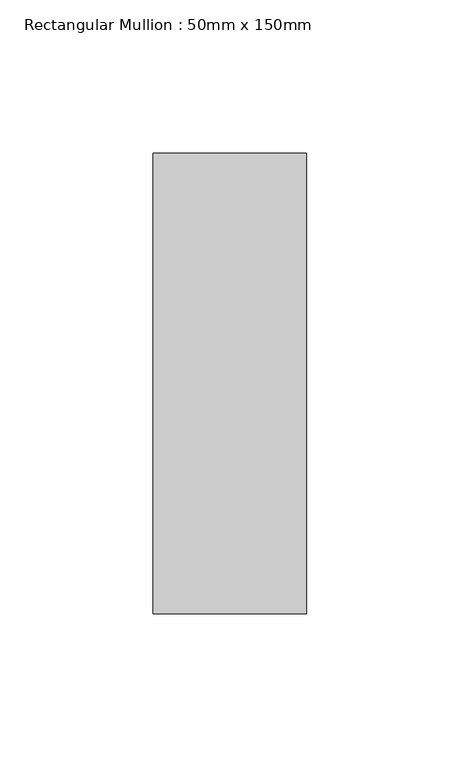
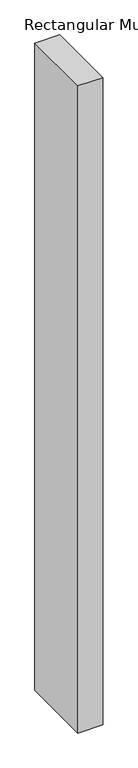
"""IFC4 building model written with IfcOpenShell, lengths in millimetres: member geometry, Rectangular Mullion : 50mm x 150mm."""

from ifc_helpers import new_model, si_unit, frame, origin, place, context, project, spatial, polyline, outline, extrude, source, transform, mapped, element, save


def rectangular_mullion_50mm_x_150mm_d2149c14(model_context):
    return source(origin(), model_context, "Body", "SweptSolid", [
        extrude(outline(polyline([(0.0, 75.0), (0.0, -75.0), (-50.0, -75.0), (-50.0, 75.0), (0.0, 75.0)])), frame((0.0, 0.0, -1376.272727), z_axis=(0.0, 0.0, 1.0), x_axis=(1.0, 0.0, 0.0)), (0.0, 0.0, 1.0), 1376.272727),
    ])


if __name__ == "__main__":
    model = new_model("IFC4")
    model_context = context("Model", 3, world=origin())
    ifc_project = project(units=[si_unit("LENGTHUNIT", "METRE", prefix="MILLI")], contexts=[model_context])
    site = spatial("IfcSite", under=ifc_project)
    building = spatial("IfcBuilding", under=site)
    placement = place(None, origin())
    rectangular_mullion_50mm_x_150mm_shape = rectangular_mullion_50mm_x_150mm_d2149c14(model_context)
    element("IfcMember", 1, ObjectType="Rectangular Mullion : 50mm x 150mm", at=placement, inside=building, context=model_context, shape_type="MappedRepresentation", body=[
        mapped(rectangular_mullion_50mm_x_150mm_shape, transform((0.0, 0.0, 0.0), x_axis=(1.0, 0.0, 0.0), y_axis=(0.0, 1.0, 0.0), z_axis=(0.0, 0.0, 1.0))),
    ])
    save(model, "model.ifc")

# Revit data of these elements
# Type "Rectangular Mullion : 50mm x 150mm"
#   built-in parameter 1007304 = 0.492126 (stored number, unit not read)
#   built-in parameter 1007301 = 0.082021 (stored number, unit not read)
#   built-in parameter 1007300 = 0.082021 (stored number, unit not read)
# Element 1 (IfcMember, "Rectangular Mullion : 50mm x 150mm")
#   Materials on its faces: "Aluminum"
# Materials
#   "Aluminum": class "Metal", colour RGB 244 244 244, transparency 0, Description = "Aluminum 6061", Cost = 0
